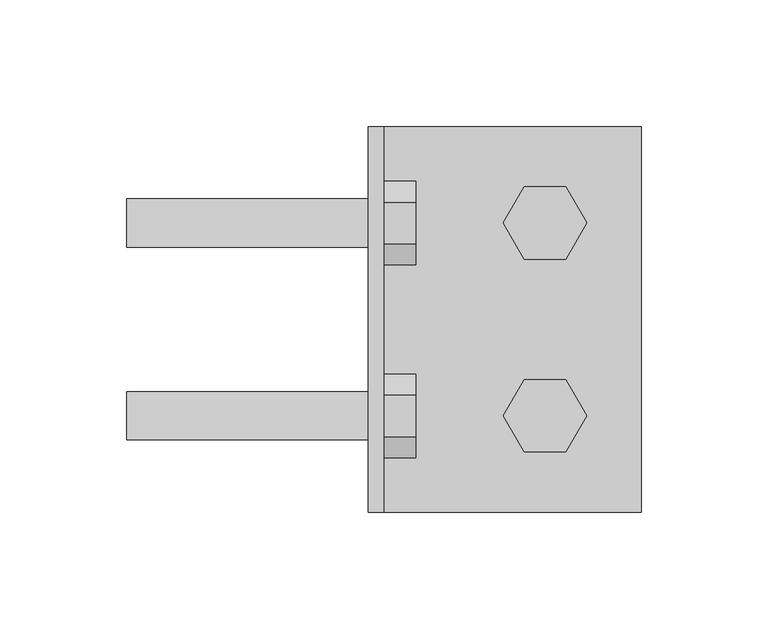
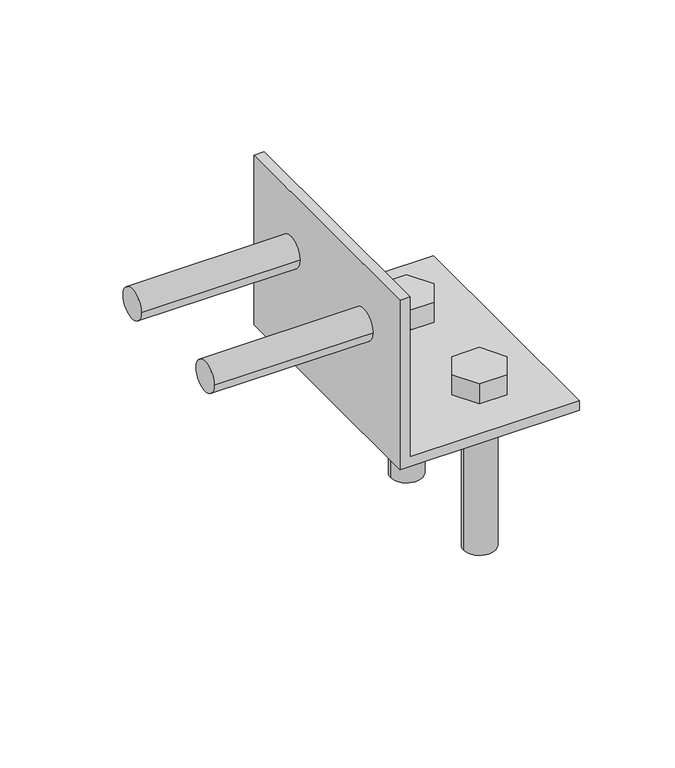
"""IFC4 building model written with IfcOpenShell, lengths in millimetres: fastener geometry, SIMPSON - HLPC/HLGPC Heavy Angles and Gussets : SIMPSON -HL46 - 6 X 4.25 - .75 Bolt - HDG."""

from ifc_helpers import new_model, si_unit, point, frame, frame_2d, origin, place, context, project, spatial, polyline, circle_curve, trimmed, segment, composite_curve, outline, extrude, source, transform, mapped, element, save
from ifc_brep_helpers import plane_surface, revolved_surface, advanced_brep


def fastener_2769678c(model_context):
    return source(origin(), model_context, "Body", "SolidModel", [
        extrude(outline(composite_curve([segment(trimmed(circle_curve(frame_2d((-38.1, 69.85)), 9.525), [point((-47.625, 69.85))], [point((-28.575, 69.85))], False, "CARTESIAN"), True, "CONTINUOUS"), segment(trimmed(circle_curve(frame_2d((-38.1, 69.85)), 9.525), [point((-28.575, 69.85))], [point((-47.625, 69.85))], False, "CARTESIAN"), True, "CONTINUOUS")], self_intersect=False)), frame((-95.5476562, 0.0, 0.0), z_axis=(1.0, 0.0, 0.0), x_axis=(0.0, 1.0, 0.0)), (0.0, 0.0, 1.0), 101.6),
        extrude(outline(polyline([(-54.5977839, 69.85), (-46.348892, 84.1375), (-29.851108, 84.1375), (-21.6022161, 69.85), (-29.851108, 55.5625), (-46.348892, 55.5625), (-54.5977839, 69.85)])), frame((6.0523438, 0.0, 0.0), z_axis=(1.0, 0.0, 0.0), x_axis=(0.0, 1.0, 0.0)), (0.0, 0.0, 1.0), 12.7),
        extrude(outline(composite_curve([segment(trimmed(circle_curve(frame_2d((38.1, 69.85)), 9.525), [point((28.575, 69.85))], [point((47.625, 69.85))], False, "CARTESIAN"), True, "CONTINUOUS"), segment(trimmed(circle_curve(frame_2d((38.1, 69.85)), 9.525), [point((47.625, 69.85))], [point((28.575, 69.85))], False, "CARTESIAN"), True, "CONTINUOUS")], self_intersect=False)), frame((-95.5476562, 0.0, 0.0), z_axis=(1.0, 0.0, 0.0), x_axis=(0.0, 1.0, 0.0)), (0.0, 0.0, 1.0), 101.6),
        extrude(outline(polyline([(21.6022161, 69.85), (29.851108, 84.1375), (46.348892, 84.1375), (54.5977839, 69.85), (46.348892, 55.5625), (29.851108, 55.5625), (21.6022161, 69.85)])), frame((6.0523438, 0.0, 0.0), z_axis=(1.0, 0.0, 0.0), x_axis=(0.0, 1.0, 0.0)), (0.0, 0.0, 1.0), 12.7),
        extrude(outline(composite_curve([segment(trimmed(circle_curve(frame_2d((69.85, 38.1)), 9.525), [point((60.325, 38.1))], [point((79.375, 38.1))], False, "CARTESIAN"), True, "CONTINUOUS"), segment(trimmed(circle_curve(frame_2d((69.85, 38.1)), 9.525), [point((79.375, 38.1))], [point((60.325, 38.1))], False, "CARTESIAN"), True, "CONTINUOUS")], self_intersect=False)), frame((0.0, 0.0, -95.5476563), z_axis=(0.0, 0.0, 1.0), x_axis=(1.0, 0.0, 0.0)), (0.0, 0.0, 1.0), 101.6),
        extrude(outline(polyline([(53.3522161, 38.1), (61.601108, 52.3875), (78.098892, 52.3875), (86.3477839, 38.1), (78.098892, 23.8125), (61.601108, 23.8125), (53.3522161, 38.1)])), frame((0.0, 0.0, 6.0523437), z_axis=(0.0, 0.0, 1.0), x_axis=(1.0, 0.0, 0.0)), (0.0, 0.0, 1.0), 12.7),
        extrude(outline(composite_curve([segment(trimmed(circle_curve(frame_2d((69.85, -38.1)), 9.525), [point((60.325, -38.1))], [point((79.375, -38.1))], False, "CARTESIAN"), True, "CONTINUOUS"), segment(trimmed(circle_curve(frame_2d((69.85, -38.1)), 9.525), [point((79.375, -38.1))], [point((60.325, -38.1))], False, "CARTESIAN"), True, "CONTINUOUS")], self_intersect=False)), frame((0.0, 0.0, -95.5476563), z_axis=(0.0, 0.0, 1.0), x_axis=(1.0, 0.0, 0.0)), (0.0, 0.0, 1.0), 101.6),
        extrude(outline(polyline([(53.3522161, -38.1), (61.601108, -23.8125), (78.098892, -23.8125), (86.3477839, -38.1), (78.098892, -52.3875), (61.601108, -52.3875), (53.3522161, -38.1)])), frame((0.0, 0.0, 6.0523437), z_axis=(0.0, 0.0, 1.0), x_axis=(1.0, 0.0, 0.0)), (0.0, 0.0, 1.0), 12.7),
        advanced_brep(
        [(6.0523438, 76.2, 107.95), (6.0523438, -76.2, 107.95), (6.0523438, -76.2, 6.0523437), (6.0523438, 76.2, 6.0523437), (6.0523438, -28.575, 69.85), (6.0523438, -47.625, 69.85), (6.0523438, 47.625, 69.85), (6.0523438, 28.575, 69.85), (0.0, -76.2, 107.95), (0.0, 76.2, 107.95), (0.0, 76.2, 0.0), (0.0, -76.2, 0.0), (0.0, -47.625, 69.85), (0.0, -28.575, 69.85), (0.0, 28.575, 69.85), (0.0, 47.625, 69.85), (107.95, -76.2, 0.0), (107.95, -76.2, 6.0523437), (107.95, 76.2, 6.0523437), (107.95, 76.2, 0.0), (79.375, -38.1, 6.0523437), (60.325, -38.1, 6.0523437), (79.375, 38.1, 6.0523437), (60.325, 38.1, 6.0523437), (60.325, -38.1, 0.0), (79.375, -38.1, 0.0), (60.325, 38.1, 0.0), (79.375, 38.1, 0.0)],
        [
            (0, 1),
            (1, 2),
            (2, 3),
            (3, 0),
            (4, 5, circle_curve(frame((6.0523438, -38.1, 69.85), z_axis=(-1.0, 0.0, 0.0), x_axis=(0.0, 1.0, 0.0)), 9.525)),
            (5, 4, circle_curve(frame((6.0523438, -38.1, 69.85), z_axis=(-1.0, 0.0, 0.0), x_axis=(0.0, 1.0, 0.0)), 9.525)),
            (6, 7, circle_curve(frame((6.0523438, 38.1, 69.85), z_axis=(-1.0, 0.0, 0.0), x_axis=(0.0, 1.0, 0.0)), 9.525)),
            (7, 6, circle_curve(frame((6.0523438, 38.1, 69.85), z_axis=(-1.0, 0.0, 0.0), x_axis=(0.0, 1.0, 0.0)), 9.525)),
            (8, 9),
            (9, 10),
            (10, 11),
            (11, 8),
            (12, 13, circle_curve(frame((0.0, -38.1, 69.85), z_axis=(1.0, 0.0, 0.0), x_axis=(0.0, 1.0, 0.0)), 9.525)),
            (13, 12, circle_curve(frame((0.0, -38.1, 69.85), z_axis=(1.0, 0.0, 0.0), x_axis=(0.0, 1.0, 0.0)), 9.525)),
            (14, 15, circle_curve(frame((0.0, 38.1, 69.85), z_axis=(1.0, 0.0, 0.0), x_axis=(0.0, 1.0, 0.0)), 9.525)),
            (15, 14, circle_curve(frame((0.0, 38.1, 69.85), z_axis=(1.0, 0.0, 0.0), x_axis=(0.0, 1.0, 0.0)), 9.525)),
            (0, 9),
            (8, 1),
            (11, 16),
            (16, 17),
            (17, 2),
            (3, 18),
            (18, 19),
            (19, 10),
            (17, 18),
            (20, 21, circle_curve(frame((69.85, -38.1, 6.0523437), z_axis=(0.0, 0.0, -1.0), x_axis=(1.0, 0.0, 0.0)), 9.525)),
            (21, 20, circle_curve(frame((69.85, -38.1, 6.0523437), z_axis=(0.0, 0.0, -1.0), x_axis=(1.0, 0.0, 0.0)), 9.525)),
            (22, 23, circle_curve(frame((69.85, 38.1, 6.0523437), z_axis=(0.0, 0.0, -1.0), x_axis=(1.0, 0.0, 0.0)), 9.525)),
            (23, 22, circle_curve(frame((69.85, 38.1, 6.0523437), z_axis=(0.0, 0.0, -1.0), x_axis=(1.0, 0.0, 0.0)), 9.525)),
            (19, 16),
            (24, 25, circle_curve(frame((69.85, -38.1, 0.0), z_axis=(0.0, 0.0, 1.0), x_axis=(1.0, 0.0, 0.0)), 9.525)),
            (25, 24, circle_curve(frame((69.85, -38.1, 0.0), z_axis=(0.0, 0.0, 1.0), x_axis=(1.0, 0.0, 0.0)), 9.525)),
            (26, 27, circle_curve(frame((69.85, 38.1, 0.0), z_axis=(0.0, 0.0, 1.0), x_axis=(1.0, 0.0, 0.0)), 9.525)),
            (27, 26, circle_curve(frame((69.85, 38.1, 0.0), z_axis=(0.0, 0.0, 1.0), x_axis=(1.0, 0.0, 0.0)), 9.525)),
            (20, 25),
            (24, 21),
            (22, 27),
            (26, 23),
            (4, 13),
            (12, 5),
            (6, 15),
            (14, 7),
        ],
        [
            plane_surface(frame((6.0523438, -76.2, 107.95), z_axis=(1.0, 0.0, 0.0), x_axis=(0.0, -1.0, 0.0))),
            plane_surface(frame((0.0, -76.2, 107.95), z_axis=(-1.0, 0.0, 0.0), x_axis=(0.0, 1.0, 0.0))),
            plane_surface(frame((6.0523438, 76.2, 107.95), z_axis=(0.0, 0.0, 1.0), x_axis=(-1.0, 0.0, 0.0))),
            plane_surface(frame((6.0523438, -76.2, 107.95), z_axis=(0.0, -1.0, 0.0), x_axis=(-1.0, 0.0, 0.0))),
            plane_surface(frame((6.0523438, 76.2, 6.0523437), z_axis=(0.0, 1.0, 0.0), x_axis=(-1.0, 0.0, 0.0))),
            plane_surface(frame((0.0, 76.2, 6.0523437), z_axis=(0.0, 0.0, 1.0), x_axis=(-1.0, 0.0, 0.0))),
            plane_surface(frame((0.0, 76.2, 0.0), z_axis=(0.0, 0.0, -1.0), x_axis=(1.0, 0.0, 0.0))),
            plane_surface(frame((107.95, -76.2, 6.0523437), z_axis=(1.0, 0.0, 0.0), x_axis=(0.0, 0.0, -1.0))),
            revolved_surface(polyline([(79.375, -38.1, 6.0523437), (79.375, -38.1, 0.0)]), (69.85, -38.1, 0.0), (0.0, 0.0, 1.0)),
            revolved_surface(polyline([(79.375, 38.1, 6.0523437), (79.375, 38.1, 0.0)]), (69.85, 38.1, 0.0), (0.0, 0.0, 1.0)),
            revolved_surface(polyline([(6.0523438, -28.575000000000003, 69.85), (0.0, -28.575000000000003, 69.85)]), (0.0, -38.1, 69.85), (1.0, 0.0, 0.0)),
            revolved_surface(polyline([(6.0523438, 47.625, 69.85), (0.0, 47.625, 69.85)]), (0.0, 38.1, 69.85), (1.0, 0.0, 0.0)),
        ],
        [
            (0, [[1, 2, 3, 4], [5, 6], [7, 8]]),
            (1, [[9, 10, 11, 12], [13, 14], [15, 16]]),
            (2, [[-1, 17, -9, 18]]),
            (3, [[-2, -18, -12, 19, 20, 21]]),
            (4, [[-4, 22, 23, 24, -10, -17]]),
            (5, [[25, -22, -3, -21], [26, 27], [28, 29]]),
            (6, [[30, -19, -11, -24], [31, 32], [33, 34]]),
            (7, [[-25, -20, -30, -23]]),
            (8, [[35, -31, 36, -26]]),
            (8, [[-35, -27, -36, -32]]),
            (9, [[37, -33, 38, -28]]),
            (9, [[-37, -29, -38, -34]]),
            (10, [[39, -13, 40, -5]]),
            (10, [[-39, -6, -40, -14]]),
            (11, [[41, -15, 42, -7]]),
            (11, [[-41, -8, -42, -16]]),
        ],
    ),
    ])


if __name__ == "__main__":
    model = new_model("IFC4")
    model_context = context("Model", 3, world=origin())
    ifc_project = project(units=[si_unit("LENGTHUNIT", "METRE", prefix="MILLI")], contexts=[model_context])
    site = spatial("IfcSite", under=ifc_project)
    building = spatial("IfcBuilding", under=site)
    placement = place(None, origin())
    fastener_shape = fastener_2769678c(model_context)
    element("IfcFastener", 1, ObjectType="SIMPSON - HLPC/HLGPC Heavy Angles and Gussets : SIMPSON -HL46 - 6 X 4.25 - .75 Bolt - HDG", at=placement, inside=building, context=model_context, shape_type="MappedRepresentation", body=[
        mapped(fastener_shape, transform((0.0, 0.0, 0.0), x_axis=(1.0, 0.0, 0.0), y_axis=(0.0, 1.0, 0.0), z_axis=(0.0, 0.0, 1.0))),
    ])
    save(model, "model.ifc")

# Revit data of these elements
# Type "SIMPSON - HLPC/HLGPC Heavy Angles and Gussets : SIMPSON -HL46 - 6 X 4.25 - .75 Bolt - HDG"
#   URL = "https://www.strongtie.com/classiccollection_architecturalproductsgroup/hlpc-hlgpc_productgroup_wcc/p/hlpc.hlgpc"
#   L = 0' - 6"
#   Hole Radius = 0' - 0 3/8"
#   D4 = 0' - 5"
#   D2 = 0' - 3"
#   D1 = 0' - 1 1/2"
#   D3 = 0' - 2 3/4"
#   Ga. = 0' - 0 61/256"
#   W1 & W2 = 0' - 4 1/4"
#   Default Elevation = 4' - 0"
#   Bolt Visibility - 3B = no
#   Bolt Visibility - 3A = no
#   Bolt Visibility - 2B = no
#   Bolt Visibility - 2A = yes
#   Bolt Visibility - 1B = no
#   Bolt Visibility - 1A = yes
#   Bolt Visibility = yes
#   Bolt Size = element 1298415
# Element 1 (IfcFastener, "SIMPSON - HLPC/HLGPC Heavy Angles and Gussets : SIMPSON -HL46 - 6 X 4.25 - .75 Bolt - HDG")
#   Materials on its faces: "1\" GALV. LAG BOLT (LENGTH = 1/2\" SHY OF GLULAM DEPTH) -  (GALV. THRU BOLT IF PLATE ON OPP. SIDE OF STRUCT MEMBER)"
# Materials
#   "1\" GALV. LAG BOLT (LENGTH = 1/2\" SHY OF GLULAM DEPTH) -  (GALV. THRU BOLT IF PLATE ON OPP. SIDE OF STRUCT MEMBER)": class "Generic", colour RGB 120 120 120, transparency 0, Cost = 0
